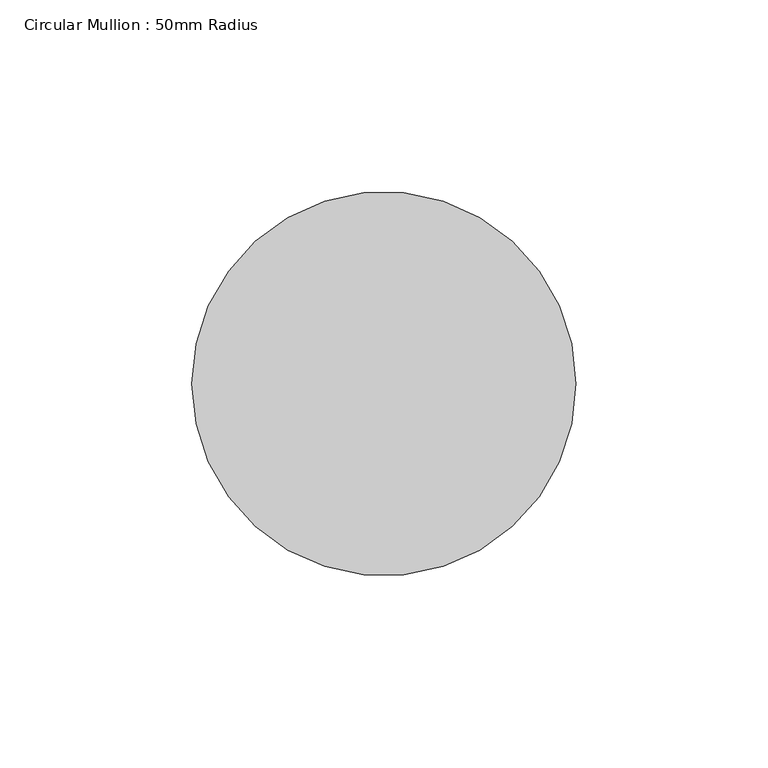
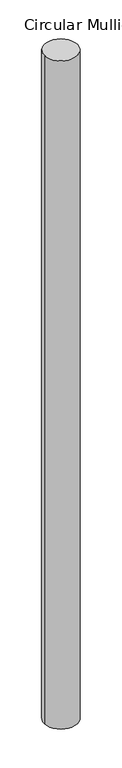
"""IFC4 building model written with IfcOpenShell, lengths in millimetres: member geometry, Circular Mullion : 50mm Radius."""

from ifc_helpers import new_model, si_unit, point, frame, frame_2d, origin, place, context, project, spatial, circle_curve, trimmed, segment, composite_curve, outline, extrude, source, transform, mapped, element, save


def circular_mullion_50mm_radius_18762c8d(model_context):
    return source(origin(), model_context, "Body", "SweptSolid", [
        extrude(outline(composite_curve([segment(trimmed(circle_curve(frame_2d((-50.0, 0.0)), 50.0), [point((0.0, 0.0))], [point((-100.0, 0.0))], False, "CARTESIAN"), True, "CONTINUOUS"), segment(trimmed(circle_curve(frame_2d((-50.0, 0.0)), 50.0), [point((-100.0, 0.0))], [point((0.0, 0.0))], False, "CARTESIAN"), True, "CONTINUOUS")], self_intersect=False)), frame((0.0, 0.0, -2125.0181559), z_axis=(0.0, 0.0, 1.0), x_axis=(1.0, 0.0, 0.0)), (0.0, 0.0, 1.0), 2125.0181559),
    ])


if __name__ == "__main__":
    model = new_model("IFC4")
    model_context = context("Model", 3, world=origin())
    ifc_project = project(units=[si_unit("LENGTHUNIT", "METRE", prefix="MILLI")], contexts=[model_context])
    site = spatial("IfcSite", under=ifc_project)
    building = spatial("IfcBuilding", under=site)
    placement = place(None, origin())
    circular_mullion_50mm_radius_shape = circular_mullion_50mm_radius_18762c8d(model_context)
    element("IfcMember", 1, ObjectType="Circular Mullion : 50mm Radius", at=placement, inside=building, context=model_context, shape_type="MappedRepresentation", body=[
        mapped(circular_mullion_50mm_radius_shape, transform((0.0, 0.0, 0.0), x_axis=(1.0, 0.0, 0.0), y_axis=(0.0, 1.0, 0.0), z_axis=(0.0, 0.0, 1.0))),
    ])
    save(model, "model.ifc")

# Revit data of these elements
# Type "Circular Mullion : 50mm Radius"
#   built-in parameter 1007350 = 0.164042 (stored number, unit not read)
# Element 1 (IfcMember, "Circular Mullion : 50mm Radius")
#   Materials on its faces: "Aluminium"
# Materials
#   "Aluminium": class "Metal", colour RGB 247 247 247, transparency 0, Description = "Aluminium 6061", Cost = 0
